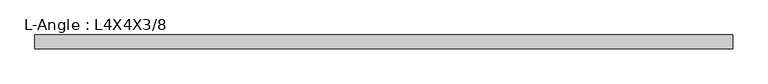
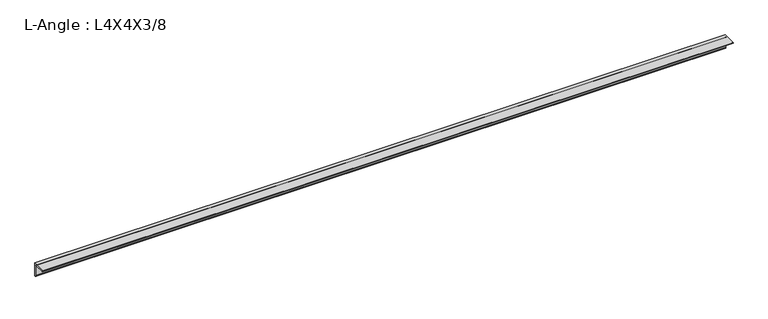
"""IFC4 building model written with IfcOpenShell, lengths in millimetres: beam geometry, L-Angle : L4X4X3/8."""

from ifc_helpers import new_model, si_unit, point, frame, frame_2d, origin, place, context, project, spatial, polyline, circle_curve, trimmed, segment, composite_curve, outline, extrude, source, transform, mapped, element, save


def l_angle_l4x4x3_8_32984166(model_context):
    return source(origin(), model_context, "Body", "SweptSolid", [
        extrude(outline(composite_curve([segment(polyline([(28.702, 28.702), (28.702, -72.898)]), True, "CONTINUOUS"), segment(trimmed(circle_curve(frame_2d((28.702, -63.373)), 9.525), [point((28.702, -72.898))], [point((19.177, -63.373))], False, "CARTESIAN"), True, "CONTINUOUS"), segment(polyline([(19.177, -63.373), (19.177, 9.652)]), True, "CONTINUOUS"), segment(trimmed(circle_curve(frame_2d((9.652, 9.652)), 9.525), [point((19.177, 9.652))], [point((9.652, 19.177))], True, "CARTESIAN"), True, "CONTINUOUS"), segment(polyline([(9.652, 19.177), (-63.373, 19.177)]), True, "CONTINUOUS"), segment(trimmed(circle_curve(frame_2d((-63.373, 28.702)), 9.525), [point((-63.373, 19.177))], [point((-72.898, 28.702))], False, "CARTESIAN"), True, "CONTINUOUS"), segment(polyline([(-72.898, 28.702), (28.702, 28.702)]), True, "CONTINUOUS")], self_intersect=False)), frame((-2565.4, 0.0, 0.0), z_axis=(1.0, 0.0, 0.0), x_axis=(0.0, 1.0, 0.0)), (0.0, 0.0, 1.0), 5118.0999994),
    ])


if __name__ == "__main__":
    model = new_model("IFC4")
    model_context = context("Model", 3, world=origin())
    ifc_project = project(units=[si_unit("LENGTHUNIT", "METRE", prefix="MILLI")], contexts=[model_context])
    site = spatial("IfcSite", under=ifc_project)
    building = spatial("IfcBuilding", under=site)
    placement = place(None, origin())
    l_angle_l4x4x3_8_shape = l_angle_l4x4x3_8_32984166(model_context)
    element("IfcBeam", 1, ObjectType="L-Angle : L4X4X3/8", at=placement, inside=building, context=model_context, shape_type="MappedRepresentation", body=[
        mapped(l_angle_l4x4x3_8_shape, transform((0.0, 0.0, 0.0), x_axis=(1.0, 0.0, 0.0), y_axis=(0.0, 1.0, 0.0), z_axis=(0.0, 0.0, 1.0))),
    ])
    save(model, "model.ifc")

# Revit data of these elements
# Type "L-Angle : L4X4X3/8"
#   Assembly Code = "B10"
#   k = 0' - 0 3/4"
#   W = 9.8
#   Length [instance default] = 5' - 0"
#   b = 0' - 4"
#   d = 0' - 4"
#   t = 0' - 0 3/8"
#   x = 0' - 1.13"
#   y = 0' - 1.13"
#   A = 0.0198611 SF
#   Structural Material [instance default] = Steel ASTM A36
# Element 1 (IfcBeam, "L-Angle : L4X4X3/8")
#   Materials on its faces: "Steel ASTM A36"
# Materials
#   "Steel ASTM A36": class "Metal", colour RGB 199 199 199, transparency 0, Description = "Structural steel, ASTM A36 Grade B, mill finish", Cost = 0
